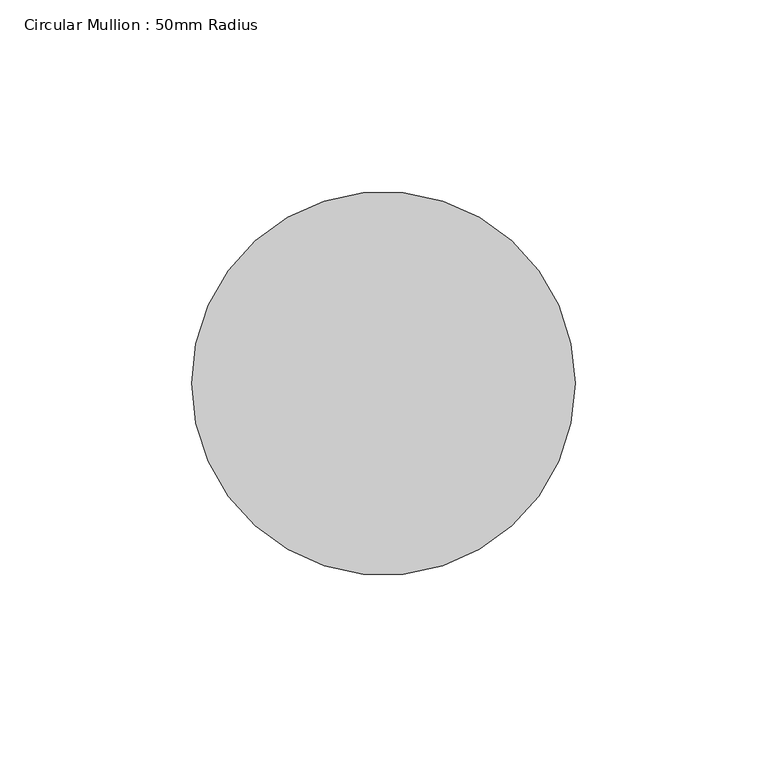
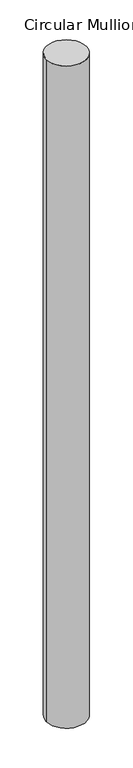
"""IFC4 building model written with IfcOpenShell, lengths in millimetres: member geometry, Circular Mullion : 50mm Radius."""

from ifc_helpers import new_model, si_unit, point, frame, origin, origin_2d, place, context, project, spatial, circle_curve, trimmed, segment, composite_curve, outline, extrude, source, transform, mapped, element, save


def circular_mullion_50mm_radius_595f0ba4(model_context):
    return source(origin(), model_context, "Body", "SweptSolid", [
        extrude(outline(composite_curve([segment(trimmed(circle_curve(origin_2d(), 50.0), [point((50.0, 0.0))], [point((-50.0, 0.0))], False, "CARTESIAN"), True, "CONTINUOUS"), segment(trimmed(circle_curve(origin_2d(), 50.0), [point((-50.0, 0.0))], [point((50.0, 0.0))], False, "CARTESIAN"), True, "CONTINUOUS")], self_intersect=False)), frame((0.0, 0.0, -1757.2387965), z_axis=(0.0, 0.0, 1.0), x_axis=(1.0, 0.0, 0.0)), (0.0, 0.0, 1.0), 1757.2387965),
    ])


if __name__ == "__main__":
    model = new_model("IFC4")
    model_context = context("Model", 3, world=origin())
    ifc_project = project(units=[si_unit("LENGTHUNIT", "METRE", prefix="MILLI")], contexts=[model_context])
    site = spatial("IfcSite", under=ifc_project)
    building = spatial("IfcBuilding", under=site)
    placement = place(None, origin())
    circular_mullion_50mm_radius_shape = circular_mullion_50mm_radius_595f0ba4(model_context)
    element("IfcMember", 1, ObjectType="Circular Mullion : 50mm Radius", at=placement, inside=building, context=model_context, shape_type="MappedRepresentation", body=[
        mapped(circular_mullion_50mm_radius_shape, transform((0.0, 0.0, 0.0), x_axis=(1.0, 0.0, 0.0), y_axis=(0.0, 1.0, 0.0), z_axis=(0.0, 0.0, 1.0))),
    ])
    save(model, "model.ifc")

# Revit data of these elements
# Type "Circular Mullion : 50mm Radius"
#   built-in parameter 1007350 = 0.164042 (stored number, unit not read)
# Element 1 (IfcMember, "Circular Mullion : 50mm Radius")
#   Materials on its faces: "Aluminium"
# Materials
#   "Aluminium": class "Metal", colour RGB 247 247 247, transparency 0, Description = "Aluminium 6061", Cost = 0
